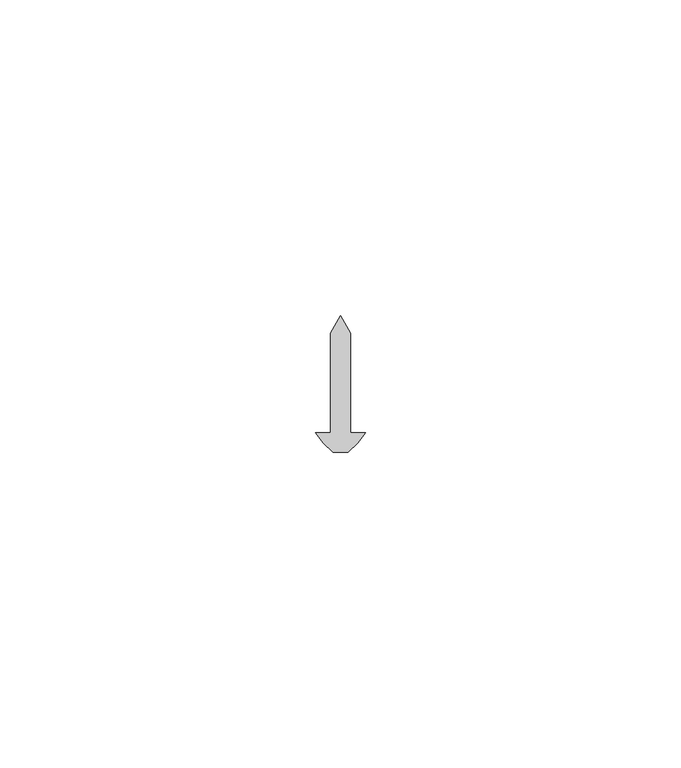
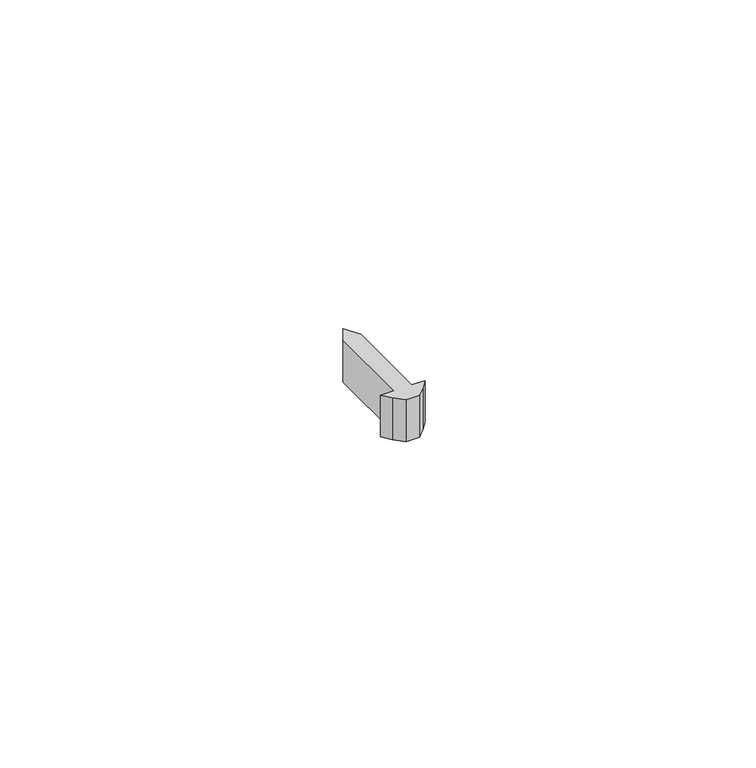
"""IFC4 building model written with IfcOpenShell, lengths in millimetres: proxy geometry, Generic Models 7:Generic Models 1:3:Generic Models 1:3 : Generic Models 7:Generic Models 1:305549:3:Generic Models 1:3:Generic Models 1:3 : Generic Models 7:Generic Models 1:305549:3 : Generic Models 7:Generic Models 1:3:Generic Models 1:3 : Generic Models 7:Generic Models 1:305549:301244:43 : Generic Models 7:Generic Models 1:3:Generic Models 1:3 : Generic Models 7:Generic Models 1:305549:3:Generic Models 1:3:Generic Models 1:3 : Generic Models 7:Generic Models 1:305549:3 : Generic Models 7:Generic Models 1:3:Generic Models 1:3 : Generic Models 7:Generic Models 1:305549:301244:308848."""

import ifcopenshell
import ifcopenshell.guid

model = None  # the IFC model being written
_history = None  # IfcOwnerHistory: only IFC2X3 demands one
_inside = {}  # id of a spatial element -> (the spatial element, [elements in it])
_under = {}  # id of a project, library or spatial element -> (it, [spatial elements below it])
_declared = {}  # id of a project -> (the project, [libraries it declares])
_typed = {}  # id of a type object -> (the type object, [elements of that type])
_made_of = {}  # id of a material, layer set ... -> (it, [elements and type objects made of it])


def new_model(schema):
    """Start an empty IFC model of exactly this schema.

    Asked for "IFC4X3", IfcOpenShell would pick the latest addendum, in which some entities
    have other attributes; the version numbers below select the first issue.
    IFC2X3 requires an IfcOwnerHistory on every rooted entity: one is made here for all.
    """
    global model, _history
    if schema == "IFC4X3":
        model = ifcopenshell.file(schema_version=(4, 3, 0, 0))
    else:
        model = ifcopenshell.file(schema=schema)
    _inside.clear()
    _under.clear()
    _declared.clear()
    _typed.clear()
    _made_of.clear()
    _history = None
    if model.schema == "IFC2X3":
        org = make("IfcOrganization", Name="unknown")
        user = make(
            "IfcPersonAndOrganization",
            ThePerson=make("IfcPerson", FamilyName="unknown"),
            TheOrganization=org,
        )
        app = make(
            "IfcApplication",
            ApplicationDeveloper=org,
            Version="unknown",
            ApplicationFullName="unknown",
            ApplicationIdentifier="unknown",
        )
        _history = make(
            "IfcOwnerHistory",
            OwningUser=user,
            OwningApplication=app,
            ChangeAction="ADDED",
            CreationDate=0,
        )
    return model


def make(cls, **values):
    """One entity of the class cls with the attributes given. An attribute that is None is left unset."""
    return model.create_entity(
        cls, **{name: value for name, value in values.items() if value is not None}
    )


def rooted(cls, **values):
    """An entity with a GlobalId (a new one), such as an element, a storey or a relation."""
    return make(cls, GlobalId=ifcopenshell.guid.new(), OwnerHistory=_history, **values)


def si_unit(unit_type, name, prefix=None):
    """IfcSIUnit, for example si_unit("LENGTHUNIT", "METRE", prefix="MILLI")."""
    return make("IfcSIUnit", UnitType=unit_type, Prefix=prefix, Name=name)


def assignment(units):
    """IfcUnitAssignment: the units of a project."""
    return None if units is None else make("IfcUnitAssignment", Units=units)


def point(xyz):
    """IfcCartesianPoint."""
    return None if xyz is None else make("IfcCartesianPoint", Coordinates=xyz)


def direction(xyz):
    """IfcDirection."""
    return None if xyz is None else make("IfcDirection", DirectionRatios=xyz)


def frame(location, z_axis=None, x_axis=None):
    """IfcAxis2Placement3D, a coordinate frame: its origin and axes. An axis left out is left unset."""
    return make(
        "IfcAxis2Placement3D",
        Location=point(location),
        Axis=direction(z_axis),
        RefDirection=direction(x_axis),
    )


def origin():
    """The frame at (0, 0, 0) with its axes left unset."""
    return frame((0.0, 0.0, 0.0))


def place(relative_to, where):
    """IfcLocalPlacement: puts the frame where relative to a parent placement (None: the world)."""
    return make(
        "IfcLocalPlacement", PlacementRelTo=relative_to, RelativePlacement=where
    )


def context(
    kind, dimensions, precision=None, world=None, true_north=None, identifier=None
):
    """IfcGeometricRepresentationContext, for example the 3D "Model" context."""
    return make(
        "IfcGeometricRepresentationContext",
        ContextIdentifier=identifier,
        ContextType=kind,
        CoordinateSpaceDimension=dimensions,
        Precision=precision,
        WorldCoordinateSystem=world,
        TrueNorth=true_north,
    )


def project(units=None, contexts=None):
    """IfcProject with its units and contexts."""
    return rooted(
        "IfcProject",
        Name="project",
        RepresentationContexts=contexts,
        UnitsInContext=assignment(units),
    )


def spatial(cls, under=None, at=None, **own):
    """A site, building, storey or space (cls), placed at a placement, below another one or the project."""
    s = rooted(cls, ObjectPlacement=at, **own)
    if under is not None:
        _under.setdefault(under.id(), (under, []))[1].append(s)
    return s


def polyline(points):
    """IfcPolyline through the points."""
    return make("IfcPolyline", Points=[point(p) for p in points])


def outline(outer, holes=None, kind="AREA"):
    """IfcArbitraryClosedProfileDef: a profile drawn as a closed curve; with holes, ...WithVoids."""
    if holes is None:
        return make("IfcArbitraryClosedProfileDef", ProfileType=kind, OuterCurve=outer)
    return make(
        "IfcArbitraryProfileDefWithVoids",
        ProfileType=kind,
        OuterCurve=outer,
        InnerCurves=holes,
    )


def extrude(swept, where, along, depth):
    """IfcExtrudedAreaSolid: the profile swept, set in the frame where, extruded along a direction by depth."""
    return make(
        "IfcExtrudedAreaSolid",
        SweptArea=swept,
        Position=where,
        ExtrudedDirection=direction(along),
        Depth=depth,
    )


def shape(context_of_items, identifier, shape_type, items):
    """IfcShapeRepresentation: the items that make up one representation, for example the "Body"."""
    return make(
        "IfcShapeRepresentation",
        ContextOfItems=context_of_items,
        RepresentationIdentifier=identifier,
        RepresentationType=shape_type,
        Items=items,
    )


def source(mapping_origin, context_of_items, identifier, shape_type, items):
    """IfcRepresentationMap: a shape defined once, which mapped items show again and again."""
    return make(
        "IfcRepresentationMap",
        MappingOrigin=mapping_origin,
        MappedRepresentation=shape(context_of_items, identifier, shape_type, items),
    )


def transform(
    local_origin,
    x_axis=None,
    y_axis=None,
    z_axis=None,
    scale=None,
    scale2=None,
    scale3=None,
    uniform=True,
):
    """IfcCartesianTransformationOperator3D, or its non-uniform kind. x_axis, y_axis, z_axis: its Axis1, 2, 3."""
    if uniform:
        return make(
            "IfcCartesianTransformationOperator3D",
            Axis1=direction(x_axis),
            Axis2=direction(y_axis),
            LocalOrigin=point(local_origin),
            Scale=scale,
            Axis3=direction(z_axis),
        )
    return make(
        "IfcCartesianTransformationOperator3DnonUniform",
        Axis1=direction(x_axis),
        Axis2=direction(y_axis),
        LocalOrigin=point(local_origin),
        Scale=scale,
        Axis3=direction(z_axis),
        Scale2=scale2,
        Scale3=scale3,
    )


def mapped(mapping_source, mapping_target):
    """IfcMappedItem: shows the shape of a source again, moved by a transform."""
    return make(
        "IfcMappedItem", MappingSource=mapping_source, MappingTarget=mapping_target
    )


def made_of(thing, what):
    """Note that an element or type object is made of a material, layer set ...; save() writes the relation."""
    if what is not None:
        _made_of.setdefault(what.id(), (what, []))[1].append(thing)
    return thing


def element(
    cls,
    number,
    at=None,
    inside=None,
    cuts=None,
    type_object=None,
    material=None,
    context=None,
    identifier="Body",
    shape_type=None,
    held_by="IfcProductDefinitionShape",
    body=None,
    shapes=None,
    **own,
):
    """One element of the class cls, such as IfcWall. Its Tag is "e" and its number.

    at: its placement. inside: the storey or other place that contains it. cuts: it is an
    opening in that element (IfcRelVoidsElement). A single representation is given by context,
    identifier, shape_type and body (its items); several are given by shapes. held_by: the class
    of the entity that holds the representations. save() writes the other relations.
    """
    e = rooted(cls, Tag="e%d" % number, ObjectPlacement=at, **own)
    if body is not None:
        shapes = [shape(context, identifier, shape_type, body)]
    if shapes is not None:
        e.Representation = make(held_by, Representations=shapes)
    if inside is not None:
        _inside.setdefault(inside.id(), (inside, []))[1].append(e)
    if cuts is not None:
        rooted(
            "IfcRelVoidsElement", RelatingBuildingElement=cuts, RelatedOpeningElement=e
        )
    if type_object is not None:
        _typed.setdefault(type_object.id(), (type_object, []))[1].append(e)
    return made_of(e, material)


def aggregate(whole, parts):
    """IfcRelAggregates: a whole, such as a stair, and the parts it consists of."""
    return rooted("IfcRelAggregates", RelatingObject=whole, RelatedObjects=parts)


def save(model, path):
    """Write the relations noted so far, then the file.

    IfcRelAggregates (storeys below a building ...), IfcRelContainedInSpatialStructure (elements
    in a storey), IfcRelDefinesByType, IfcRelAssociatesMaterial and IfcRelDeclares: one each for
    every whole, place, type object, material and project.
    """
    for whole, parts in _under.values():
        aggregate(whole, parts)
    for where, things in _inside.values():
        rooted(
            "IfcRelContainedInSpatialStructure",
            RelatedElements=things,
            RelatingStructure=where,
        )
    for kind, things in _typed.values():
        rooted("IfcRelDefinesByType", RelatedObjects=things, RelatingType=kind)
    for what, things in _made_of.values():
        rooted("IfcRelAssociatesMaterial", RelatedObjects=things, RelatingMaterial=what)
    for by, libraries in _declared.values():
        rooted("IfcRelDeclares", RelatingContext=by, RelatedDefinitions=libraries)
    model.write(path)


def generic_models_27c82eae(model_context):
    return source(origin(), model_context, "Body", "SweptSolid", [
        extrude(outline(polyline([(560672.0492239, -579084.8288841), (560672.0492239, -579069.0196286), (560673.6367239, -579066.2699979), (560675.2242239, -579069.0196286), (560675.2242239, -579084.8288841), (560677.6054739, -579084.8288841), (560676.3872784, -579086.3559421), (560674.8353882, -579087.9078323), (560672.4380597, -579087.9078323), (560670.8861695, -579086.3559421), (560669.6679739, -579084.8288841), (560672.0492239, -579084.8288841)])), frame((0.0, 0.0, 4907.75625), z_axis=(0.0, 0.0, 1.0), x_axis=(1.0, 0.0, 0.0)), (0.0, 0.0, 1.0), 7.9375),
    ])


if __name__ == "__main__":
    model = new_model("IFC4")
    model_context = context("Model", 3, world=origin())
    ifc_project = project(units=[si_unit("LENGTHUNIT", "METRE", prefix="MILLI")], contexts=[model_context])
    site = spatial("IfcSite", under=ifc_project)
    building = spatial("IfcBuilding", under=site)
    placement = place(None, origin())
    generic_models_shape = generic_models_27c82eae(model_context)
    element("IfcBuildingElementProxy", 1, Name="Generic Models 7:Generic Models 1:3:Generic Models 1:3 : Generic Models 7:Generic Models 1:305549:3:Generic Models 1:3:Generic Models 1:3 : Generic Models 7:Generic Models 1:305549:3 : Generic Models 7:Generic Models 1:3:Generic Models 1:3 : Generic Models 7:Generic Models 1:305549:301244:43 : Generic Models 7:Generic Models 1:3:Generic Models 1:3 : Generic Models 7:Generic Models 1:305549:3:Generic Models 1:3:Generic Models 1:3 : Generic Models 7:Generic Models 1:305549:3 : Generic Models 7:Generic Models 1:3:Generic Models 1:3 : Generic Models 7:Generic Models 1:305549:301244:308848", ObjectType="Generic Models 7:Generic Models 1:3:Generic Models 1:3 : Generic Models 7:Generic Models 1:305549:3:Generic Models 1:3:Generic Models 1:3 : Generic Models 7:Generic Models 1:305549:3 : Generic Models 7:Generic Models 1:3:Generic Models 1:3 : Generic Models 7:Generic Models 1:305549:301244:43 : Generic Models 7:Generic Models 1:3:Generic Models 1:3 : Generic Models 7:Generic Models 1:305549:3:Generic Models 1:3:Generic Models 1:3 : Generic Models 7:Generic Models 1:305549:3 : Generic Models 7:Generic Models 1:3:Generic Models 1:3 : Generic Models 7:Generic Models 1:305549:301244:308848", at=placement, inside=building, context=model_context, shape_type="MappedRepresentation", body=[
        mapped(generic_models_shape, transform((0.0, 0.0, 0.0), x_axis=(1.0, 0.0, 0.0), y_axis=(0.0, 1.0, 0.0), z_axis=(0.0, 0.0, 1.0))),
    ])
    save(model, "model.ifc")

# Revit data of these elements
# Type "Generic Models 7:Generic Models 1:3:Generic Models 1:3 : Generic Models 7:Generic Models 1:305549:3:Generic Models 1:3:Generic Models 1:3 : Generic Models 7:Generic Models 1:305549:3 : Generic Models 7:Generic Models 1:3:Generic Models 1:3 : Generic Models 7:Generic Models 1:305549:301244:43 : Generic Models 7:Generic Models 1:3:Generic Models 1:3 : Generic Models 7:Generic Models 1:305549:3:Generic Models 1:3:Generic Models 1:3 : Generic Models 7:Generic Models 1:305549:3 : Generic Models 7:Generic Models 1:3:Generic Models 1:3 : Generic Models 7:Generic Models 1:305549:301244:308848"
#   NameOverride = "Generic Models 7:Generic Models 1:3:Generic Models 1:3 : Generic Models 7:Generic Models 1:305549:3:Generic Models 1:3:Generic Models 1:3 : Generic Models 7:Generic Models 1:305549:3 : Generic Models 7:Generic Models 1:3:Generic Models 1:3 : Generic Models 7:Generic Models 1:305549:301244:308848"
#   ObjectTypeOverride = "Generic Models 1:3:Generic Models 1:3 : Generic Models 7:Generic Models 1:305549:3 : Generic Models 7:Generic Models 1:3:Generic Models 1:3 : Generic Models 7:Generic Models 1:305549:301244"
#   Reference = "Generic Models 1"
#   Tag = "308848"
# Element 1 (IfcBuildingElementProxy, "Generic Models 7:Generic Models 1:3:Generic Models 1:3 : Generic Models 7:Generic Models 1:305549:3:Generic Models 1:3:Generic Models 1:3 : Generic Models 7:Generic Models 1:305549:3 : Generic Models 7:Generic Models 1:3:Generic Models 1:3 : Generic Models 7:Generic Models 1:305549:301244:43 : Generic Models 7:Generic Models 1:3:Generic Models 1:3 : Generic Models 7:Generic Models 1:305549:3:Generic Models 1:3:Generic Models 1:3 : Generic Models 7:Generic Models 1:305549:3 : Generic Models 7:Generic Models 1:3:Generic Models 1:3 : Generic Models 7:Generic Models 1:305549:301244:308848")
#   Materials on its faces: "FASTENERS (T.B.D)"
# Materials
#   "FASTENERS (T.B.D)": class "Generic", colour RGB 120 120 120, transparency 0, Cost = 0
